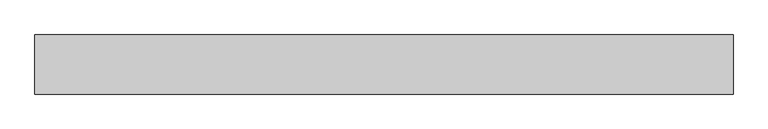
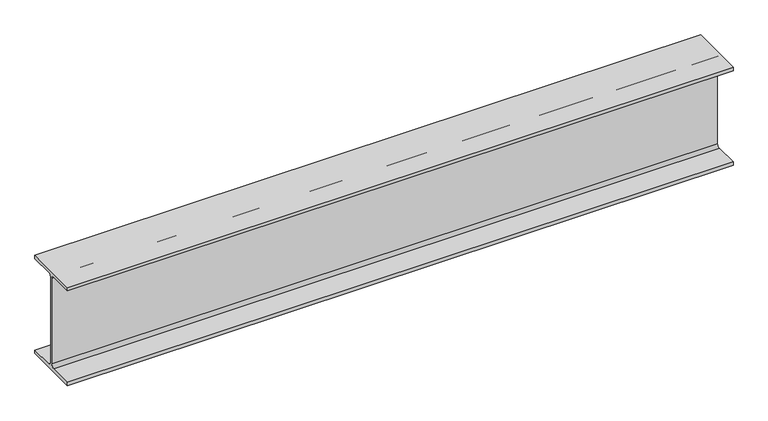
"""IFC4 building model written with IfcOpenShell, lengths in millimetres: beam geometry, Old_Steel Beam_H-KSD3502 : H_SB_ASB_H-200×200x8x12."""

import ifcopenshell
import ifcopenshell.guid

model = None  # the IFC model being written
_history = None  # IfcOwnerHistory: only IFC2X3 demands one
_inside = {}  # id of a spatial element -> (the spatial element, [elements in it])
_under = {}  # id of a project, library or spatial element -> (it, [spatial elements below it])
_declared = {}  # id of a project -> (the project, [libraries it declares])
_typed = {}  # id of a type object -> (the type object, [elements of that type])
_made_of = {}  # id of a material, layer set ... -> (it, [elements and type objects made of it])


def new_model(schema):
    """Start an empty IFC model of exactly this schema.

    Asked for "IFC4X3", IfcOpenShell would pick the latest addendum, in which some entities
    have other attributes; the version numbers below select the first issue.
    IFC2X3 requires an IfcOwnerHistory on every rooted entity: one is made here for all.
    """
    global model, _history
    if schema == "IFC4X3":
        model = ifcopenshell.file(schema_version=(4, 3, 0, 0))
    else:
        model = ifcopenshell.file(schema=schema)
    _inside.clear()
    _under.clear()
    _declared.clear()
    _typed.clear()
    _made_of.clear()
    _history = None
    if model.schema == "IFC2X3":
        org = make("IfcOrganization", Name="unknown")
        user = make(
            "IfcPersonAndOrganization",
            ThePerson=make("IfcPerson", FamilyName="unknown"),
            TheOrganization=org,
        )
        app = make(
            "IfcApplication",
            ApplicationDeveloper=org,
            Version="unknown",
            ApplicationFullName="unknown",
            ApplicationIdentifier="unknown",
        )
        _history = make(
            "IfcOwnerHistory",
            OwningUser=user,
            OwningApplication=app,
            ChangeAction="ADDED",
            CreationDate=0,
        )
    return model


def make(cls, **values):
    """One entity of the class cls with the attributes given. An attribute that is None is left unset."""
    return model.create_entity(
        cls, **{name: value for name, value in values.items() if value is not None}
    )


def rooted(cls, **values):
    """An entity with a GlobalId (a new one), such as an element, a storey or a relation."""
    return make(cls, GlobalId=ifcopenshell.guid.new(), OwnerHistory=_history, **values)


def si_unit(unit_type, name, prefix=None):
    """IfcSIUnit, for example si_unit("LENGTHUNIT", "METRE", prefix="MILLI")."""
    return make("IfcSIUnit", UnitType=unit_type, Prefix=prefix, Name=name)


def assignment(units):
    """IfcUnitAssignment: the units of a project."""
    return None if units is None else make("IfcUnitAssignment", Units=units)


def point(xyz):
    """IfcCartesianPoint."""
    return None if xyz is None else make("IfcCartesianPoint", Coordinates=xyz)


def direction(xyz):
    """IfcDirection."""
    return None if xyz is None else make("IfcDirection", DirectionRatios=xyz)


def frame(location, z_axis=None, x_axis=None):
    """IfcAxis2Placement3D, a coordinate frame: its origin and axes. An axis left out is left unset."""
    return make(
        "IfcAxis2Placement3D",
        Location=point(location),
        Axis=direction(z_axis),
        RefDirection=direction(x_axis),
    )


def frame_2d(location, x_axis=None):
    """IfcAxis2Placement2D, a coordinate frame in the plane: its origin and x axis."""
    return make(
        "IfcAxis2Placement2D", Location=point(location), RefDirection=direction(x_axis)
    )


def origin():
    """The frame at (0, 0, 0) with its axes left unset."""
    return frame((0.0, 0.0, 0.0))


def place(relative_to, where):
    """IfcLocalPlacement: puts the frame where relative to a parent placement (None: the world)."""
    return make(
        "IfcLocalPlacement", PlacementRelTo=relative_to, RelativePlacement=where
    )


def context(
    kind, dimensions, precision=None, world=None, true_north=None, identifier=None
):
    """IfcGeometricRepresentationContext, for example the 3D "Model" context."""
    return make(
        "IfcGeometricRepresentationContext",
        ContextIdentifier=identifier,
        ContextType=kind,
        CoordinateSpaceDimension=dimensions,
        Precision=precision,
        WorldCoordinateSystem=world,
        TrueNorth=true_north,
    )


def project(units=None, contexts=None):
    """IfcProject with its units and contexts."""
    return rooted(
        "IfcProject",
        Name="project",
        RepresentationContexts=contexts,
        UnitsInContext=assignment(units),
    )


def spatial(cls, under=None, at=None, **own):
    """A site, building, storey or space (cls), placed at a placement, below another one or the project."""
    s = rooted(cls, ObjectPlacement=at, **own)
    if under is not None:
        _under.setdefault(under.id(), (under, []))[1].append(s)
    return s


def polyline(points):
    """IfcPolyline through the points."""
    return make("IfcPolyline", Points=[point(p) for p in points])


def circle_curve(where, radius):
    """IfcCircle in the frame where."""
    return make("IfcCircle", Position=where, Radius=radius)


def trimmed(basis, trim1, trim2, sense, master):
    """IfcTrimmedCurve: the piece of a basis curve between two trims."""
    return make(
        "IfcTrimmedCurve",
        BasisCurve=basis,
        Trim1=trim1,
        Trim2=trim2,
        SenseAgreement=sense,
        MasterRepresentation=master,
    )


def segment(curve, same_sense, transition):
    """IfcCompositeCurveSegment."""
    return make(
        "IfcCompositeCurveSegment",
        Transition=transition,
        SameSense=same_sense,
        ParentCurve=curve,
    )


def composite_curve(segments, self_intersect=None):
    """IfcCompositeCurve: segments joined end to end."""
    return make("IfcCompositeCurve", Segments=segments, SelfIntersect=self_intersect)


def outline(outer, holes=None, kind="AREA"):
    """IfcArbitraryClosedProfileDef: a profile drawn as a closed curve; with holes, ...WithVoids."""
    if holes is None:
        return make("IfcArbitraryClosedProfileDef", ProfileType=kind, OuterCurve=outer)
    return make(
        "IfcArbitraryProfileDefWithVoids",
        ProfileType=kind,
        OuterCurve=outer,
        InnerCurves=holes,
    )


def extrude(swept, where, along, depth):
    """IfcExtrudedAreaSolid: the profile swept, set in the frame where, extruded along a direction by depth."""
    return make(
        "IfcExtrudedAreaSolid",
        SweptArea=swept,
        Position=where,
        ExtrudedDirection=direction(along),
        Depth=depth,
    )


def shape(context_of_items, identifier, shape_type, items):
    """IfcShapeRepresentation: the items that make up one representation, for example the "Body"."""
    return make(
        "IfcShapeRepresentation",
        ContextOfItems=context_of_items,
        RepresentationIdentifier=identifier,
        RepresentationType=shape_type,
        Items=items,
    )


def source(mapping_origin, context_of_items, identifier, shape_type, items):
    """IfcRepresentationMap: a shape defined once, which mapped items show again and again."""
    return make(
        "IfcRepresentationMap",
        MappingOrigin=mapping_origin,
        MappedRepresentation=shape(context_of_items, identifier, shape_type, items),
    )


def transform(
    local_origin,
    x_axis=None,
    y_axis=None,
    z_axis=None,
    scale=None,
    scale2=None,
    scale3=None,
    uniform=True,
):
    """IfcCartesianTransformationOperator3D, or its non-uniform kind. x_axis, y_axis, z_axis: its Axis1, 2, 3."""
    if uniform:
        return make(
            "IfcCartesianTransformationOperator3D",
            Axis1=direction(x_axis),
            Axis2=direction(y_axis),
            LocalOrigin=point(local_origin),
            Scale=scale,
            Axis3=direction(z_axis),
        )
    return make(
        "IfcCartesianTransformationOperator3DnonUniform",
        Axis1=direction(x_axis),
        Axis2=direction(y_axis),
        LocalOrigin=point(local_origin),
        Scale=scale,
        Axis3=direction(z_axis),
        Scale2=scale2,
        Scale3=scale3,
    )


def mapped(mapping_source, mapping_target):
    """IfcMappedItem: shows the shape of a source again, moved by a transform."""
    return make(
        "IfcMappedItem", MappingSource=mapping_source, MappingTarget=mapping_target
    )


def made_of(thing, what):
    """Note that an element or type object is made of a material, layer set ...; save() writes the relation."""
    if what is not None:
        _made_of.setdefault(what.id(), (what, []))[1].append(thing)
    return thing


def element(
    cls,
    number,
    at=None,
    inside=None,
    cuts=None,
    type_object=None,
    material=None,
    context=None,
    identifier="Body",
    shape_type=None,
    held_by="IfcProductDefinitionShape",
    body=None,
    shapes=None,
    **own,
):
    """One element of the class cls, such as IfcWall. Its Tag is "e" and its number.

    at: its placement. inside: the storey or other place that contains it. cuts: it is an
    opening in that element (IfcRelVoidsElement). A single representation is given by context,
    identifier, shape_type and body (its items); several are given by shapes. held_by: the class
    of the entity that holds the representations. save() writes the other relations.
    """
    e = rooted(cls, Tag="e%d" % number, ObjectPlacement=at, **own)
    if body is not None:
        shapes = [shape(context, identifier, shape_type, body)]
    if shapes is not None:
        e.Representation = make(held_by, Representations=shapes)
    if inside is not None:
        _inside.setdefault(inside.id(), (inside, []))[1].append(e)
    if cuts is not None:
        rooted(
            "IfcRelVoidsElement", RelatingBuildingElement=cuts, RelatedOpeningElement=e
        )
    if type_object is not None:
        _typed.setdefault(type_object.id(), (type_object, []))[1].append(e)
    return made_of(e, material)


def aggregate(whole, parts):
    """IfcRelAggregates: a whole, such as a stair, and the parts it consists of."""
    return rooted("IfcRelAggregates", RelatingObject=whole, RelatedObjects=parts)


def save(model, path):
    """Write the relations noted so far, then the file.

    IfcRelAggregates (storeys below a building ...), IfcRelContainedInSpatialStructure (elements
    in a storey), IfcRelDefinesByType, IfcRelAssociatesMaterial and IfcRelDeclares: one each for
    every whole, place, type object, material and project.
    """
    for whole, parts in _under.values():
        aggregate(whole, parts)
    for where, things in _inside.values():
        rooted(
            "IfcRelContainedInSpatialStructure",
            RelatedElements=things,
            RelatingStructure=where,
        )
    for kind, things in _typed.values():
        rooted("IfcRelDefinesByType", RelatedObjects=things, RelatingType=kind)
    for what, things in _made_of.values():
        rooted("IfcRelAssociatesMaterial", RelatedObjects=things, RelatingMaterial=what)
    for by, libraries in _declared.values():
        rooted("IfcRelDeclares", RelatingContext=by, RelatedDefinitions=libraries)
    model.write(path)


def beam_cc15ee5d(model_context):
    return source(origin(), model_context, "Body", "SweptSolid", [
        extrude(outline(composite_curve([segment(polyline([(82.5, -141.5), (82.5, -151.7), (-82.5, -151.7), (-82.5, -141.5), (-11.9, -141.5)]), True, "CONTINUOUS"), segment(trimmed(circle_curve(frame_2d((-11.9, -132.6)), 8.9), [point((-11.9, -141.5))], [point((-3.0, -132.6))], True, "CARTESIAN"), True, "CONTINUOUS"), segment(polyline([(-3.0, -132.6), (-3.0, 132.6)]), True, "CONTINUOUS"), segment(trimmed(circle_curve(frame_2d((-11.9, 132.6)), 8.9), [point((-3.0, 132.6))], [point((-11.9, 141.5))], True, "CARTESIAN"), True, "CONTINUOUS"), segment(polyline([(-11.9, 141.5), (-82.5, 141.5), (-82.5, 151.7), (82.5, 151.7), (82.5, 141.5), (11.9, 141.5)]), True, "CONTINUOUS"), segment(trimmed(circle_curve(frame_2d((11.9, 132.6)), 8.9), [point((11.9, 141.5))], [point((3.0, 132.6))], True, "CARTESIAN"), True, "CONTINUOUS"), segment(polyline([(3.0, 132.6), (3.0, -132.6)]), True, "CONTINUOUS"), segment(trimmed(circle_curve(frame_2d((11.9, -132.6)), 8.9), [point((3.0, -132.6))], [point((11.9, -141.5))], True, "CARTESIAN"), True, "CONTINUOUS"), segment(polyline([(11.9, -141.5), (82.5, -141.5)]), True, "CONTINUOUS")], self_intersect=False)), frame((-921.1968525, 0.0, 0.0), z_axis=(1.0, 0.0, 0.0), x_axis=(0.0, 1.0, 0.0)), (0.0, 0.0, 1.0), 1948.528739),
    ])


if __name__ == "__main__":
    model = new_model("IFC4")
    model_context = context("Model", 3, world=origin())
    ifc_project = project(units=[si_unit("LENGTHUNIT", "METRE", prefix="MILLI")], contexts=[model_context])
    site = spatial("IfcSite", under=ifc_project)
    building = spatial("IfcBuilding", under=site)
    placement = place(None, origin())
    beam_shape = beam_cc15ee5d(model_context)
    element("IfcBeam", 1, ObjectType="Old_Steel Beam_H-KSD3502 : H_SB_ASB_H-200×200x8x12", at=placement, inside=building, context=model_context, shape_type="MappedRepresentation", body=[
        mapped(beam_shape, transform((0.0, 0.0, 0.0), x_axis=(1.0, 0.0, 0.0), y_axis=(0.0, 1.0, 0.0), z_axis=(0.0, 0.0, 1.0))),
    ])
    save(model, "model.ifc")

# Revit data of these elements
# Type "Old_Steel Beam_H-KSD3502 : H_SB_ASB_H-200×200x8x12"
#   Width = 20.0 cm
#   Web Thickness = 0.8 cm
#   Web Fillet = 1.3 cm
#   Warping Constant = 141376.0 cm⁶
#   Torsional Moment of Inertia = 26.2485 cm⁴
#   Torsional Modulus = 1.0 cm³
#   Section Area = 63.53 cm²
#   Plastic Modulus weak axis = 244.0 cm³
#   Plastic Modulus strong axis = 525.0 cm³
#   Perimeter = 1.16 m²/m
#   Nominal Weight = 49.90 kgf/m
#   Moment of Inertia weak axis = 1600.00 cm⁴
#   Moment of Inertia strong axis = 4720.00 cm⁴
#   Height = 20.0 cm
#   Flange Thickness = 1.2 cm
#   Elastic Modulus weak axis = 160.0 cm³
#   Elastic Modulus strong axis = 472.0 cm³
#   Centroid Vertical = 10.0 cm
#   Centroid Horizontal = 10.0 cm
#   Length [instance default] = 1.5240 m
#   Structural Material [instance default] = Steel, 45-345
#   Assembly Code = ""
# Element 1 (IfcBeam, "Old_Steel Beam_H-KSD3502 : H_SB_ASB_H-200×200x8x12")
#   Structural Material = none
# Materials
#   "Steel, 45-345": class "Metal", colour RGB 189 187 185, transparency 0, Description = "Steel 345 MPa", Cost = 0
